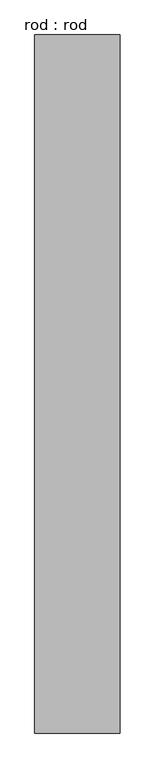
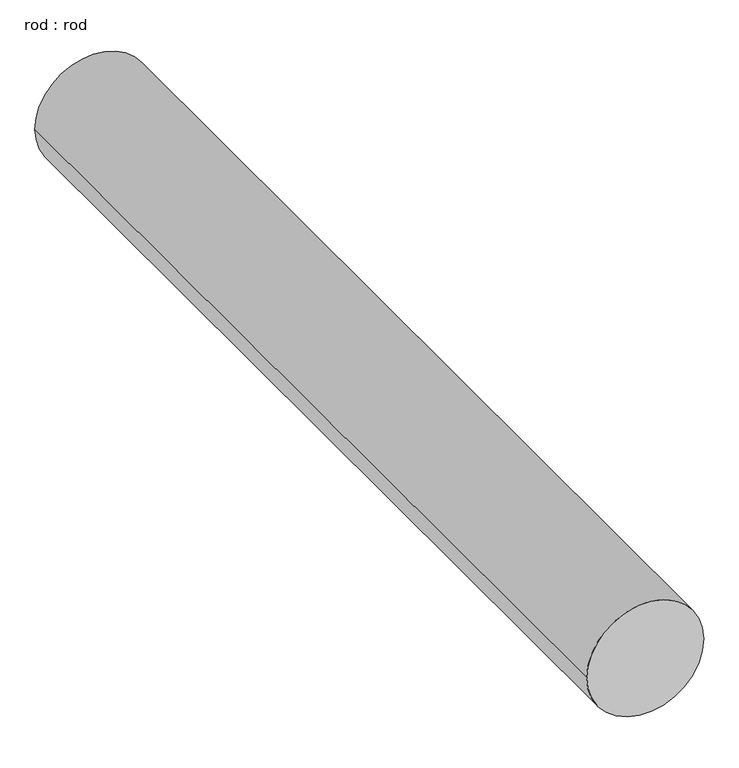
"""IFC4 building model written with IfcOpenShell, lengths in millimetres: proxy geometry, rod : rod."""

from ifc_helpers import new_model, si_unit, point, frame, frame_2d, origin, place, context, project, spatial, circle_curve, trimmed, segment, composite_curve, outline, extrude, source, transform, mapped, element, save


def rod_rod_6e68d2d4(model_context):
    return source(origin(), model_context, "Body", "SweptSolid", [
        extrude(outline(composite_curve([segment(trimmed(circle_curve(frame_2d((0.0108462, 0.0)), 200.0), [point((0.0108462, 200.0))], [point((0.0108462, -200.0))], False, "CARTESIAN"), True, "CONTINUOUS"), segment(trimmed(circle_curve(frame_2d((0.0108462, 0.0)), 200.0), [point((0.0108462, -200.0))], [point((0.0108462, 200.0))], False, "CARTESIAN"), True, "CONTINUOUS")], self_intersect=False)), frame((0.0, 2458.8000439, 0.0), z_axis=(0.0, 1.0, 0.0), x_axis=(0.0, 0.0, 1.0)), (0.0, 0.0, 1.0), 3267.8571429),
    ])


if __name__ == "__main__":
    model = new_model("IFC4")
    model_context = context("Model", 3, world=origin())
    ifc_project = project(units=[si_unit("LENGTHUNIT", "METRE", prefix="MILLI")], contexts=[model_context])
    site = spatial("IfcSite", under=ifc_project)
    building = spatial("IfcBuilding", under=site)
    placement = place(None, origin())
    rod_rod_shape = rod_rod_6e68d2d4(model_context)
    element("IfcBuildingElementProxy", 1, Name="rod : rod", ObjectType="rod : rod", at=placement, inside=building, context=model_context, shape_type="MappedRepresentation", body=[
        mapped(rod_rod_shape, transform((0.0, 0.0, 0.0), x_axis=(1.0, 0.0, 0.0), y_axis=(0.0, 1.0, 0.0), z_axis=(0.0, 0.0, 1.0))),
    ])
    save(model, "model.ifc")

# Revit data of these elements
# Type "rod : rod"
#   Default Elevation = 0
